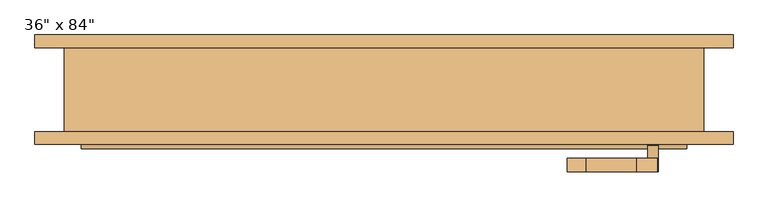
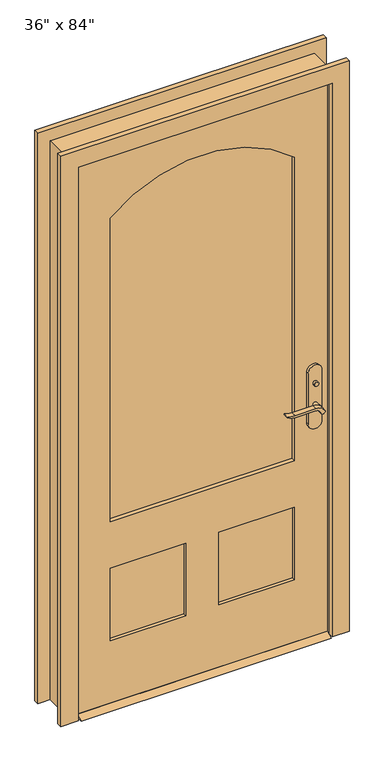
"""IFC4 building model written with IfcOpenShell, lengths in millimetres: door geometry."""

from ifc_helpers import new_model, si_unit, point, frame, frame_2d, origin, place, context, project, spatial, polyline, circle_curve, trimmed, segment, composite_curve, outline, extrude, faceted_brep, source, transform, mapped, element, save


def door_cff610c9(model_context):
    return source(origin(), model_context, "Body", "SolidModel", [
        extrude(outline(polyline([(-25.4, 12.7), (0.0, 0.0), (-85.725, 0.0), (-60.325, 12.7), (-25.4, 12.7)])), frame((-457.2, 0.0, 0.0), z_axis=(1.0, 0.0, 0.0), x_axis=(0.0, 1.0, 0.0)), (0.0, 0.0, 1.0), 914.4),
        extrude(outline(polyline([(411.4, -5.4), (411.4, -15.4), (401.4, -15.4), (401.4, -5.4), (411.4, -5.4)])), frame((0.0, 0.0, 981.9), z_axis=(0.0, 0.0, 1.0), x_axis=(1.0, 0.0, 0.0)), (0.0, 0.0, 1.0), 30.0),
        extrude(outline(composite_curve([segment(trimmed(circle_curve(frame_2d((996.9, 406.4)), 8.0), [point((996.9, 398.4))], [point((996.9, 414.4))], False, "CARTESIAN"), True, "CONTINUOUS"), segment(trimmed(circle_curve(frame_2d((996.9, 406.4)), 8.0), [point((996.9, 414.4))], [point((996.9, 398.4))], False, "CARTESIAN"), True, "CONTINUOUS")], self_intersect=False)), frame((0.0, -80.325, 0.0), z_axis=(0.0, 1.0, 0.0), x_axis=(0.0, 0.0, 1.0)), (0.0, 0.0, 1.0), 10.0),
        extrude(outline(composite_curve([segment(trimmed(circle_curve(frame_2d((897.1555521, 382.7324871)), 37.2832219), [point((919.0523287, 412.9081363))], [point((934.4, 381.0325667))], False, "CARTESIAN"), True, "CONTINUOUS"), segment(polyline([(934.4, 381.0325667), (934.4, 304.7564091)]), True, "CONTINUOUS"), segment(trimmed(circle_curve(frame_2d((1017.6850638, 304.8227909)), 83.2850902), [point((934.4, 304.7564091))], [point((939.4, 276.4))], True, "CARTESIAN"), True, "CONTINUOUS"), segment(polyline([(939.4, 276.4), (936.6135558, 276.4)]), True, "CONTINUOUS"), segment(trimmed(circle_curve(frame_2d((986.6709207, 308.3396612)), 59.3791355), [point((936.6135558, 276.4))], [point((927.4, 304.7564091))], False, "CARTESIAN"), True, "CONTINUOUS"), segment(polyline([(927.4, 304.7564091), (927.4, 381.0138099)]), True, "CONTINUOUS"), segment(trimmed(circle_curve(frame_2d((909.2738613, 381.0138099)), 18.1261387), [point((927.4, 381.0138099))], [point((914.4, 398.4))], True, "CARTESIAN"), True, "CONTINUOUS"), segment(trimmed(circle_curve(frame_2d((914.4, 406.4)), 8.0), [point((914.4, 398.4))], [point((919.0523287, 412.9081363))], False, "CARTESIAN"), True, "CONTINUOUS")], self_intersect=False)), frame((0.0, 14.6, 0.0), z_axis=(0.0, 1.0, 0.0), x_axis=(0.0, 0.0, 1.0)), (0.0, 0.0, 1.0), 20.0),
        extrude(outline(composite_curve([segment(trimmed(circle_curve(frame_2d((914.4, 406.4)), 8.0), [point((914.3999903, 398.4))], [point((919.0523287, 412.9081363))], False, "CARTESIAN"), True, "CONTINUOUS"), segment(trimmed(circle_curve(frame_2d((897.1555521, 382.7324871)), 37.2832219), [point((919.0523287, 412.9081363))], [point((934.4, 381.0325667))], False, "CARTESIAN"), True, "CONTINUOUS"), segment(polyline([(934.4, 381.0325667), (934.4, 304.7564091)]), True, "CONTINUOUS"), segment(trimmed(circle_curve(frame_2d((1017.6850638, 304.8227909)), 83.2850902), [point((934.4, 304.7564091))], [point((939.4, 276.4))], True, "CARTESIAN"), True, "CONTINUOUS"), segment(polyline([(939.4, 276.4), (936.6135558, 276.4)]), True, "CONTINUOUS"), segment(trimmed(circle_curve(frame_2d((986.6709207, 308.3396612)), 59.3791355), [point((936.6135558, 276.4))], [point((927.4, 304.7564091))], False, "CARTESIAN"), True, "CONTINUOUS"), segment(polyline([(927.4, 304.7564091), (927.4, 381.0138122)]), True, "CONTINUOUS"), segment(trimmed(circle_curve(frame_2d((909.2738682, 381.0138122)), 18.1261318), [point((927.4, 381.0138122))], [point((914.3999903, 398.4))], True, "CARTESIAN"), True, "CONTINUOUS")], self_intersect=False)), frame((0.0, -120.325, 0.0), z_axis=(0.0, 1.0, 0.0), x_axis=(0.0, 0.0, 1.0)), (0.0, 0.0, 1.0), 20.0),
        extrude(outline(composite_curve([segment(trimmed(circle_curve(frame_2d((914.4, 406.4)), 8.0), [point((914.4, 398.4))], [point((914.4, 414.4))], False, "CARTESIAN"), True, "CONTINUOUS"), segment(trimmed(circle_curve(frame_2d((914.4, 406.4)), 8.0), [point((914.4, 414.4))], [point((914.4, 398.4))], False, "CARTESIAN"), True, "CONTINUOUS")], self_intersect=False)), frame((0.0, -15.4, 0.0), z_axis=(0.0, 1.0, 0.0), x_axis=(0.0, 0.0, 1.0)), (0.0, 0.0, 1.0), 30.0),
        extrude(outline(composite_curve([segment(trimmed(circle_curve(frame_2d((914.4, 406.4)), 8.0), [point((914.4, 398.4))], [point((914.4, 414.4))], False, "CARTESIAN"), True, "CONTINUOUS"), segment(trimmed(circle_curve(frame_2d((914.4, 406.4)), 8.0), [point((914.4, 414.4))], [point((914.4, 398.4))], False, "CARTESIAN"), True, "CONTINUOUS")], self_intersect=False)), frame((0.0, -100.325, 0.0), z_axis=(0.0, 1.0, 0.0), x_axis=(0.0, 0.0, 1.0)), (0.0, 0.0, 1.0), 30.0),
        extrude(outline(composite_curve([segment(polyline([(844.4, 431.4), (1039.4, 431.4)]), True, "CONTINUOUS"), segment(trimmed(circle_curve(frame_2d((1039.4, 406.4)), 25.0), [point((1039.4, 431.4))], [point((1039.4, 381.4))], False, "CARTESIAN"), True, "CONTINUOUS"), segment(polyline([(1039.4, 381.4), (844.4, 381.4)]), True, "CONTINUOUS"), segment(trimmed(circle_curve(frame_2d((844.4, 406.4)), 25.0), [point((844.4, 381.4))], [point((844.4, 431.4))], False, "CARTESIAN"), True, "CONTINUOUS")], self_intersect=False)), frame((0.0, -25.4, 0.0), z_axis=(0.0, 1.0, 0.0), x_axis=(0.0, 0.0, 1.0)), (0.0, 0.0, 1.0), 10.0),
        extrude(outline(composite_curve([segment(polyline([(844.4, 431.4), (1039.4, 431.4)]), True, "CONTINUOUS"), segment(trimmed(circle_curve(frame_2d((1039.4, 406.4)), 25.0), [point((1039.4, 431.4))], [point((1039.4, 381.4))], False, "CARTESIAN"), True, "CONTINUOUS"), segment(polyline([(1039.4, 381.4), (844.4, 381.4)]), True, "CONTINUOUS"), segment(trimmed(circle_curve(frame_2d((844.4, 406.4)), 25.0), [point((844.4, 381.4))], [point((844.4, 431.4))], False, "CARTESIAN"), True, "CONTINUOUS")], self_intersect=False)), frame((0.0, -70.325, 0.0), z_axis=(0.0, 1.0, 0.0), x_axis=(0.0, 0.0, 1.0)), (0.0, 0.0, 1.0), 10.0),
        extrude(outline(polyline([(2133.6, -457.2), (12.7, -457.2), (12.7, 457.2), (2133.6, 457.2), (2133.6, -457.2)]), holes=[composite_curve([segment(polyline([(714.375, -336.55), (1885.95, -336.55)]), True, "CONTINUOUS"), segment(trimmed(circle_curve(frame_2d((1503.52125, 0.0)), 509.42875), [point((1885.95, -336.55))], [point((1885.95, 336.55))], True, "CARTESIAN"), True, "CONTINUOUS"), segment(polyline([(1885.95, 336.55), (714.375, 336.55), (714.375, -336.55)]), True, "CONTINUOUS")], self_intersect=False), polyline([(533.4, -60.325), (254.0, -60.325), (254.0, -336.55), (533.4, -336.55), (533.4, -60.325)]), polyline([(533.4, 336.55), (254.0, 336.55), (254.0, 60.325), (533.4, 60.325), (533.4, 336.55)])]), frame((0.0, -60.325, 0.0), z_axis=(0.0, 1.0, 0.0), x_axis=(0.0, 0.0, 1.0)), (0.0, 0.0, 1.0), 34.925),
        faceted_brep([(482.6, -60.325, 0.0), (457.2, -60.325, 0.0), (457.2, -25.4, 0.0), (444.5, -25.4, 0.0), (444.5, 9.525, 0.0), (457.2, 9.525, 0.0), (457.2, 66.675, 0.0), (482.6, 66.675, 0.0), (482.6, 66.675, 2159.0), (482.6, -60.325, 2159.0), (457.2, 66.675, 2133.6), (-457.2, 66.675, 2133.6), (-457.2, 66.675, 0.0), (-482.6, 66.675, 0.0), (-482.6, 66.675, 2159.0), (457.2, 9.525, 2133.6), (444.5, 9.525, 2120.9), (-444.5, 9.525, 2120.9), (-444.5, 9.525, 0.0), (-457.2, 9.525, 0.0), (-457.2, 9.525, 2133.6), (444.5, -25.4, 2120.9), (457.2, -25.4, 2133.6), (-457.2, -25.4, 2133.6), (-457.2, -25.4, 0.0), (-444.5, -25.4, 0.0), (-444.5, -25.4, 2120.9), (457.2, -60.325, 2133.6), (-482.6, -60.325, 2159.0), (-482.6, -60.325, 0.0), (-457.2, -60.325, 0.0), (-457.2, -60.325, 2133.6)], [[[0, 1, 2, 3, 4, 5, 6, 7]], [[7, 8, 9, 0]], [[6, 10, 11, 12, 13, 14, 8, 7]], [[5, 15, 10, 6]], [[4, 16, 17, 18, 19, 20, 15, 5]], [[3, 21, 16, 4]], [[2, 22, 23, 24, 25, 26, 21, 3]], [[1, 27, 22, 2]], [[0, 9, 28, 29, 30, 31, 27, 1]], [[8, 14, 28, 9]], [[15, 20, 11, 10]], [[21, 26, 17, 16]], [[27, 31, 23, 22]], [[29, 13, 12, 19, 18, 25, 24, 30]], [[14, 13, 29, 28]], [[20, 19, 12, 11]], [[26, 25, 18, 17]], [[31, 30, 24, 23]]]),
        extrude(outline(polyline([(-60.325, -37.0416667), (-60.325, -48.6833333), (-336.55, -48.6833333), (-336.55, -37.0416667), (-60.325, -37.0416667)])), frame((0.0, 0.0, 254.0), z_axis=(0.0, 0.0, 1.0), x_axis=(1.0, 0.0, 0.0)), (0.0, 0.0, 1.0), 279.4),
        extrude(outline(polyline([(336.55, -37.0416667), (336.55, -48.6833333), (60.325, -48.6833333), (60.325, -37.0416667), (336.55, -37.0416667)])), frame((0.0, 0.0, 254.0), z_axis=(0.0, 0.0, 1.0), x_axis=(1.0, 0.0, 0.0)), (0.0, 0.0, 1.0), 279.4),
        extrude(outline(composite_curve([segment(polyline([(714.375, -336.55), (714.375, 336.55), (1885.95, 336.55)]), True, "CONTINUOUS"), segment(trimmed(circle_curve(frame_2d((1503.52125, 0.0)), 509.42875), [point((1885.95, 336.55))], [point((1885.95, -336.55))], False, "CARTESIAN"), True, "CONTINUOUS"), segment(polyline([(1885.95, -336.55), (714.375, -336.55)]), True, "CONTINUOUS")], self_intersect=False)), frame((0.0, -46.355, 0.0), z_axis=(0.0, 1.0, 0.0), x_axis=(0.0, 0.0, 1.0)), (0.0, 0.0, 1.0), 6.985),
        extrude(outline(polyline([(0.0, -463.55), (2139.95, -463.55), (2139.95, 463.55), (0.0, 463.55), (0.0, 527.05), (2203.45, 527.05), (2203.45, -527.05), (0.0, -527.05), (0.0, -463.55)])), frame((0.0, 66.675, 0.0), z_axis=(0.0, 1.0, 0.0), x_axis=(0.0, 0.0, 1.0)), (0.0, 0.0, 1.0), 19.05),
        extrude(outline(polyline([(0.0, -463.55), (2139.95, -463.55), (2139.95, 463.55), (0.0, 463.55), (0.0, 527.05), (2203.45, 527.05), (2203.45, -527.05), (0.0, -527.05), (0.0, -463.55)])), frame((0.0, -79.375, 0.0), z_axis=(0.0, 1.0, 0.0), x_axis=(0.0, 0.0, 1.0)), (0.0, 0.0, 1.0), 19.05),
    ])


if __name__ == "__main__":
    model = new_model("IFC4")
    model_context = context("Model", 3, world=origin())
    ifc_project = project(units=[si_unit("LENGTHUNIT", "METRE", prefix="MILLI")], contexts=[model_context])
    site = spatial("IfcSite", under=ifc_project)
    building = spatial("IfcBuilding", under=site)
    placement = place(None, origin())
    door_shape = door_cff610c9(model_context)
    element("IfcDoor", 1, ObjectType="Door-Exterior-Single-Entry-Half Arch Glass-Wood_Clad : 36\" x 84\"", at=placement, inside=building, context=model_context, shape_type="MappedRepresentation", body=[
        mapped(door_shape, transform((0.0, 0.0, 0.0), x_axis=(1.0, 0.0, 0.0), y_axis=(0.0, 1.0, 0.0), z_axis=(0.0, 0.0, 1.0))),
    ])
    save(model, "model.ifc")

# Revit data of these elements
# Type "Door-Exterior-Single-Entry-Half Arch Glass-Wood_Clad : 36\" x 84\""
#   Type Mark = "x"
#   Assembly Code = "B2030100"
#   Analytic Construction = "French door, wood frame with single glass"
#   Threshold Offset [instance default] = 0' - 0 1/2"
#   Thickness = 0' - 1 3/8"
#   Thermal Resistance (R) = 0.188367 (m²·K)/W
#   Swing Angle [instance default] = 90.00°
#   Stiles = 0' - 4 3/4"
#   Rough Width = 3' - 2"
#   Rough Height = 7' - 1"
#   Radius = 1' - 8.05625"
#   Lock Rail = 0' - 7 1/8"
#   Height = 7' - 0"
#   Width = 3' - 0"
#   Heat Transfer Coefficient (U) = 5.30918 W/(m²·K)
#   Door Offset [instance default] = 0' - 0"
#   Bottom Rail = 0' - 9 1/2"
#   Threshold [instance default] = yes
#   Function = 1
#   Exterior Trim [instance default] = yes
#   Trim Material = Trim
#   Threshold Material = Trim
#   Panel Material = Trim
#   Glazing = EXISTING WINDOW
#   Frame Material = Trim
#   Door Handle Material = Trim
#   Visual Light Transmittance = 0
#   Solar Heat Gain Coefficient = 0
#   Wall Closure = (empty or 0)
#   Construction Type = (empty or 0)
# Element 1 (IfcDoor, "Door-Exterior-Single-Entry-Half Arch Glass-Wood_Clad : 36\" x 84\"")
#   Materials on its faces: "Trim", "EXISTING WINDOW"
# Materials
#   "Trim": class "Wood", colour RGB 250 251 245, transparency 0, Cost = 0
#   "EXISTING WINDOW": class "Glass", colour RGB 218 227 224, transparency 0.85, Description = "Soda Lime Glass", Cost = 0
